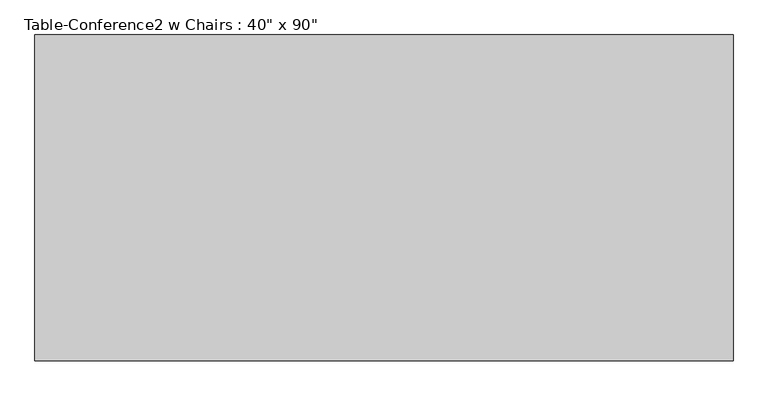
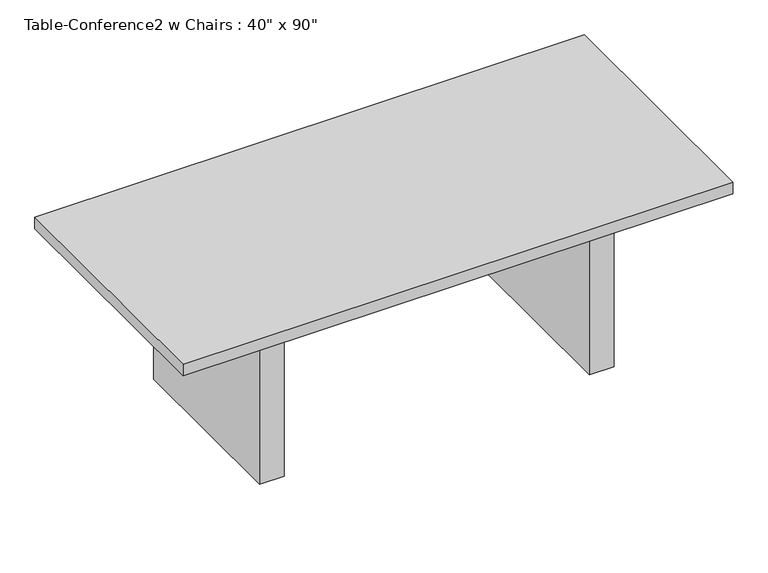
"""IFC4 building model written with IfcOpenShell, lengths in millimetres: furniture geometry."""

from ifc_helpers import new_model, si_unit, frame, origin, origin_with_axes, place, context, project, spatial, polyline, outline, extrude, source, transform, mapped, element, save


def furniture_ed4cefae(model_context):
    return source(origin(), model_context, "Body", "SweptSolid", [
        extrude(outline(polyline([(635.0, 381.0), (635.0, 342.9), (-635.0, 342.9), (-635.0, 381.0), (635.0, 381.0)])), frame((0.0, 0.0, 609.6), z_axis=(0.0, 0.0, 1.0), x_axis=(1.0, 0.0, 0.0)), (0.0, 0.0, 1.0), 101.6),
        extrude(outline(polyline([(635.0, -381.0), (-635.0, -381.0), (-635.0, -342.9), (635.0, -342.9), (635.0, -381.0)])), frame((0.0, 0.0, 609.6), z_axis=(0.0, 0.0, 1.0), x_axis=(1.0, 0.0, 0.0)), (0.0, 0.0, 1.0), 101.6),
        extrude(outline(polyline([(-635.0, -381.0), (-736.6, -381.0), (-736.6, 381.0), (-635.0, 381.0), (-635.0, -381.0)])), origin_with_axes(), (0.0, 0.0, 1.0), 711.2),
        extrude(outline(polyline([(736.6, -381.0), (635.0, -381.0), (635.0, 381.0), (736.6, 381.0), (736.6, -381.0)])), origin_with_axes(), (0.0, 0.0, 1.0), 711.2),
        extrude(outline(polyline([(1143.0, -533.4), (-1143.0, -533.4), (-1143.0, 533.4), (1143.0, 533.4), (1143.0, -533.4)])), frame((0.0, 0.0, 711.2), z_axis=(0.0, 0.0, 1.0), x_axis=(1.0, 0.0, 0.0)), (0.0, 0.0, 1.0), 50.8),
    ])


if __name__ == "__main__":
    model = new_model("IFC4")
    model_context = context("Model", 3, world=origin())
    ifc_project = project(units=[si_unit("LENGTHUNIT", "METRE", prefix="MILLI")], contexts=[model_context])
    site = spatial("IfcSite", under=ifc_project)
    building = spatial("IfcBuilding", under=site)
    placement = place(None, origin())
    furniture_shape = furniture_ed4cefae(model_context)
    element("IfcFurniture", 1, ObjectType="Table-Conference2 w Chairs : 40\" x 90\"", at=placement, inside=building, context=model_context, shape_type="MappedRepresentation", body=[
        mapped(furniture_shape, transform((0.0, 0.0, 0.0), x_axis=(1.0, 0.0, 0.0), y_axis=(0.0, 1.0, 0.0), z_axis=(0.0, 0.0, 1.0))),
    ])
    save(model, "model.ifc")

# Revit data of these elements
# Type "Table-Conference2 w Chairs : 40\" x 90\""
#   Type IfcGUID = "2u0XNFrAPALBFZCv81fqic"
#   Assembly Code = "E2020200"
#   Description = "Seating 6-8"
#   Height = 0.762 m
#   Length = 2.286 m
#   Width = 1.0668 m
#   Number Of Chairs One Side = 3
#   Number Of Chairs = 8
#   Material = Wood - Cherry
#   Default Elevation = 0
# Element 1 (IfcFurniture, "Table-Conference2 w Chairs : 40\" x 90\"")
#   Materials on its faces: "Wood - Cherry"
# Materials
#   "Wood - Cherry": class "Wood", colour RGB 226 177 128, transparency 0
